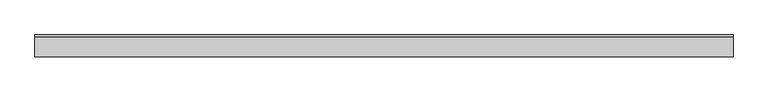
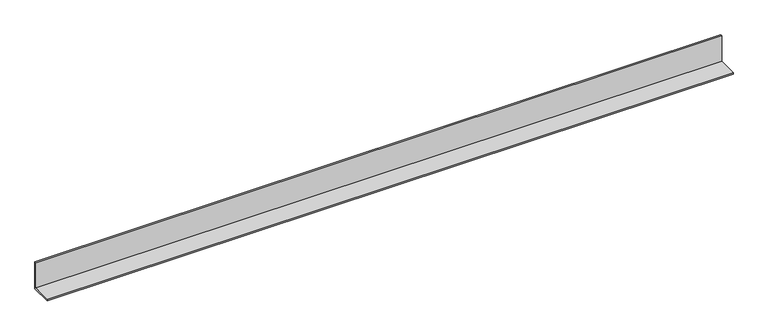
"""IFC4 building model written with IfcOpenShell, lengths in millimetres: proxy geometry, Generic Models 3:Generic Models 1:6:Generic Models 1:6 : Generic Models 3:Generic Models 1:300625:350611:Generic Models 1:6:Generic Models 1:6 : Generic Models 3:Generic Models 1:300625:350611 : Generic Models 3:Generic Models 1:6:Generic Models 1:6 : Generic Models 3:Generic Models 1:300625:350611:5 : Generic Models 3:Generic Models 1:6:Generic Models 1:6 : Generic Models 3:Generic Models 1:300625:350611:Generic Models 1:6:Generic Models 1:6 : Generic Models 3:Generic Models 1:300625:350611 : Generic Models 3:Generic Models 1:6:Generic Models 1:6 : Generic Models 3:Generic Models 1:300625:350611:301824."""

from ifc_helpers import new_model, si_unit, frame, origin, place, context, project, spatial, polyline, outline, extrude, source, transform, mapped, element, save


def generic_models_cb24bc7f(model_context):
    return source(origin(), model_context, "Body", "SweptSolid", [
        extrude(outline(polyline([(-578797.4913841, 0.0), (-578873.6913841, 0.0), (-578873.6913841, 6.35), (-578803.8413841, 6.35), (-578803.8413841, 101.6), (-578797.4913841, 101.6), (-578797.4913841, 0.0)])), frame((570452.6367239, 0.0, 0.0), z_axis=(1.0, 0.0, 0.0), x_axis=(0.0, 1.0, 0.0)), (0.0, 0.0, 1.0), 2438.4),
    ])


if __name__ == "__main__":
    model = new_model("IFC4")
    model_context = context("Model", 3, world=origin())
    ifc_project = project(units=[si_unit("LENGTHUNIT", "METRE", prefix="MILLI")], contexts=[model_context])
    site = spatial("IfcSite", under=ifc_project)
    building = spatial("IfcBuilding", under=site)
    placement = place(None, origin())
    generic_models_shape = generic_models_cb24bc7f(model_context)
    element("IfcBuildingElementProxy", 1, Name="Generic Models 3:Generic Models 1:6:Generic Models 1:6 : Generic Models 3:Generic Models 1:300625:350611:Generic Models 1:6:Generic Models 1:6 : Generic Models 3:Generic Models 1:300625:350611 : Generic Models 3:Generic Models 1:6:Generic Models 1:6 : Generic Models 3:Generic Models 1:300625:350611:5 : Generic Models 3:Generic Models 1:6:Generic Models 1:6 : Generic Models 3:Generic Models 1:300625:350611:Generic Models 1:6:Generic Models 1:6 : Generic Models 3:Generic Models 1:300625:350611 : Generic Models 3:Generic Models 1:6:Generic Models 1:6 : Generic Models 3:Generic Models 1:300625:350611:301824", ObjectType="Generic Models 3:Generic Models 1:6:Generic Models 1:6 : Generic Models 3:Generic Models 1:300625:350611:Generic Models 1:6:Generic Models 1:6 : Generic Models 3:Generic Models 1:300625:350611 : Generic Models 3:Generic Models 1:6:Generic Models 1:6 : Generic Models 3:Generic Models 1:300625:350611:5 : Generic Models 3:Generic Models 1:6:Generic Models 1:6 : Generic Models 3:Generic Models 1:300625:350611:Generic Models 1:6:Generic Models 1:6 : Generic Models 3:Generic Models 1:300625:350611 : Generic Models 3:Generic Models 1:6:Generic Models 1:6 : Generic Models 3:Generic Models 1:300625:350611:301824", at=placement, inside=building, context=model_context, shape_type="MappedRepresentation", body=[
        mapped(generic_models_shape, transform((0.0, 0.0, 0.0), x_axis=(1.0, 0.0, 0.0), y_axis=(0.0, 1.0, 0.0), z_axis=(0.0, 0.0, 1.0))),
    ])
    save(model, "model.ifc")

# Revit data of these elements
# Type "Generic Models 3:Generic Models 1:6:Generic Models 1:6 : Generic Models 3:Generic Models 1:300625:350611:Generic Models 1:6:Generic Models 1:6 : Generic Models 3:Generic Models 1:300625:350611 : Generic Models 3:Generic Models 1:6:Generic Models 1:6 : Generic Models 3:Generic Models 1:300625:350611:5 : Generic Models 3:Generic Models 1:6:Generic Models 1:6 : Generic Models 3:Generic Models 1:300625:350611:Generic Models 1:6:Generic Models 1:6 : Generic Models 3:Generic Models 1:300625:350611 : Generic Models 3:Generic Models 1:6:Generic Models 1:6 : Generic Models 3:Generic Models 1:300625:350611:301824"
#   NameOverride = "Generic Models 3:Generic Models 1:6:Generic Models 1:6 : Generic Models 3:Generic Models 1:300625:350611:Generic Models 1:6:Generic Models 1:6 : Generic Models 3:Generic Models 1:300625:350611 : Generic Models 3:Generic Models 1:6:Generic Models 1:6 : Generic Models 3:Generic Models 1:300625:350611:301824"
#   ObjectTypeOverride = "Generic Models 1:6:Generic Models 1:6 : Generic Models 3:Generic Models 1:300625:350611 : Generic Models 3:Generic Models 1:6:Generic Models 1:6 : Generic Models 3:Generic Models 1:300625:350611"
#   Reference = "Generic Models 1"
#   Tag = "301824"
